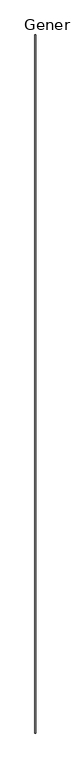
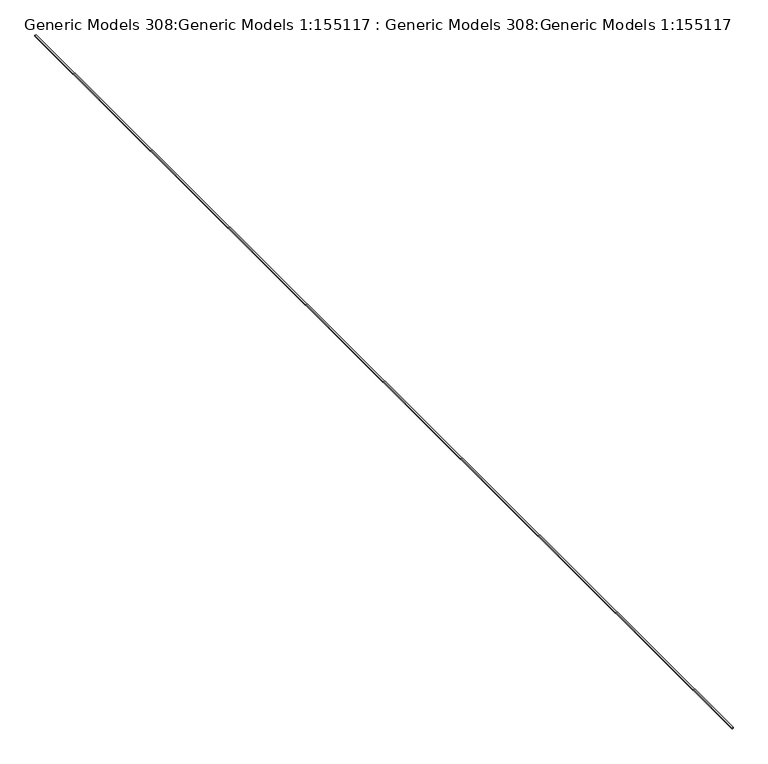
"""IFC4 building model written with IfcOpenShell, lengths in millimetres: proxy geometry, Generic Models 308:Generic Models 1:155117 : Generic Models 308:Generic Models 1:155117."""

from ifc_helpers import new_model, si_unit, point, frame, frame_2d, origin, place, context, project, spatial, polyline, circle_curve, trimmed, segment, composite_curve, outline, extrude, source, transform, mapped, element, save


def generic_models_308_generic_models_1_155117_generic_models_2615cf28(model_context):
    return source(origin(), model_context, "Body", "SweptSolid", [
        extrude(outline(composite_curve([segment(trimmed(circle_curve(frame_2d((82.029481, 6835.653213)), 8.620055), [point((76.2, 6842.003213))], [point((76.2, 6829.303213))], True, "CARTESIAN"), True, "CONTINUOUS"), segment(polyline([(76.2, 6829.303213), (66.675, 6829.303213)]), True, "CONTINUOUS"), segment(trimmed(circle_curve(frame_2d((72.504481, 6835.653213)), 8.620055), [point((66.675, 6829.303213))], [point((66.675, 6842.003213))], False, "CARTESIAN"), True, "CONTINUOUS"), segment(polyline([(66.675, 6842.003213), (76.2, 6842.003213)]), True, "CONTINUOUS")], self_intersect=False)), frame((0.0, 8191.2927644, 0.0), z_axis=(0.0, 1.0, 0.0), x_axis=(0.0, 0.0, 1.0)), (0.0, 0.0, 1.0), 12344.4),
    ])


if __name__ == "__main__":
    model = new_model("IFC4")
    model_context = context("Model", 3, world=origin())
    ifc_project = project(units=[si_unit("LENGTHUNIT", "METRE", prefix="MILLI")], contexts=[model_context])
    site = spatial("IfcSite", under=ifc_project)
    building = spatial("IfcBuilding", under=site)
    placement = place(None, origin())
    generic_models_308_generic_models_1_155117_generic_models_shape = generic_models_308_generic_models_1_155117_generic_models_2615cf28(model_context)
    element("IfcBuildingElementProxy", 1, Name="Generic Models 308:Generic Models 1:155117 : Generic Models 308:Generic Models 1:155117", ObjectType="Generic Models 308:Generic Models 1:155117 : Generic Models 308:Generic Models 1:155117", at=placement, inside=building, context=model_context, shape_type="MappedRepresentation", body=[
        mapped(generic_models_308_generic_models_1_155117_generic_models_shape, transform((0.0, 0.0, 0.0), x_axis=(1.0, 0.0, 0.0), y_axis=(0.0, 1.0, 0.0), z_axis=(0.0, 0.0, 1.0))),
    ])
    save(model, "model.ifc")

# Revit data of these elements
# Type "Generic Models 308:Generic Models 1:155117 : Generic Models 308:Generic Models 1:155117"
#   NameOverride = "Generic Models 308:Generic Models 1:155117"
#   ObjectTypeOverride = "Generic Models 308:Generic Models 1"
#   Reference = "Generic Models 1"
#   Category = "Generic Models"
#   Tag = "155117"
# Element 1 (IfcBuildingElementProxy, "Generic Models 308:Generic Models 1:155117 : Generic Models 308:Generic Models 1:155117")
#   Materials on its faces: "_SEALANT JOINT 27113"
# Materials
#   "_SEALANT JOINT 27113": class "Unassigned", colour RGB 190 220 196, transparency 0
